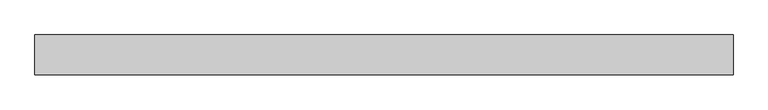
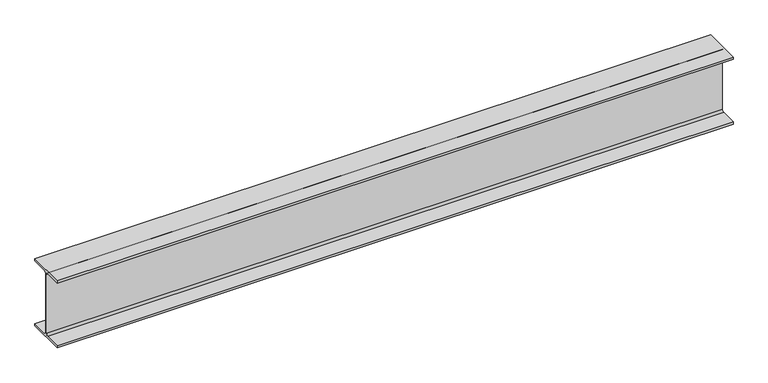
"""IFC4 building model written with IfcOpenShell, lengths in millimetres: beam geometry, Steel Beam_H-KSD3502 : H_SB_ASB_H-250x125x6x9."""

import ifcopenshell
import ifcopenshell.guid

model = None  # the IFC model being written
_history = None  # IfcOwnerHistory: only IFC2X3 demands one
_inside = {}  # id of a spatial element -> (the spatial element, [elements in it])
_under = {}  # id of a project, library or spatial element -> (it, [spatial elements below it])
_declared = {}  # id of a project -> (the project, [libraries it declares])
_typed = {}  # id of a type object -> (the type object, [elements of that type])
_made_of = {}  # id of a material, layer set ... -> (it, [elements and type objects made of it])


def new_model(schema):
    """Start an empty IFC model of exactly this schema.

    Asked for "IFC4X3", IfcOpenShell would pick the latest addendum, in which some entities
    have other attributes; the version numbers below select the first issue.
    IFC2X3 requires an IfcOwnerHistory on every rooted entity: one is made here for all.
    """
    global model, _history
    if schema == "IFC4X3":
        model = ifcopenshell.file(schema_version=(4, 3, 0, 0))
    else:
        model = ifcopenshell.file(schema=schema)
    _inside.clear()
    _under.clear()
    _declared.clear()
    _typed.clear()
    _made_of.clear()
    _history = None
    if model.schema == "IFC2X3":
        org = make("IfcOrganization", Name="unknown")
        user = make(
            "IfcPersonAndOrganization",
            ThePerson=make("IfcPerson", FamilyName="unknown"),
            TheOrganization=org,
        )
        app = make(
            "IfcApplication",
            ApplicationDeveloper=org,
            Version="unknown",
            ApplicationFullName="unknown",
            ApplicationIdentifier="unknown",
        )
        _history = make(
            "IfcOwnerHistory",
            OwningUser=user,
            OwningApplication=app,
            ChangeAction="ADDED",
            CreationDate=0,
        )
    return model


def make(cls, **values):
    """One entity of the class cls with the attributes given. An attribute that is None is left unset."""
    return model.create_entity(
        cls, **{name: value for name, value in values.items() if value is not None}
    )


def rooted(cls, **values):
    """An entity with a GlobalId (a new one), such as an element, a storey or a relation."""
    return make(cls, GlobalId=ifcopenshell.guid.new(), OwnerHistory=_history, **values)


def si_unit(unit_type, name, prefix=None):
    """IfcSIUnit, for example si_unit("LENGTHUNIT", "METRE", prefix="MILLI")."""
    return make("IfcSIUnit", UnitType=unit_type, Prefix=prefix, Name=name)


def assignment(units):
    """IfcUnitAssignment: the units of a project."""
    return None if units is None else make("IfcUnitAssignment", Units=units)


def point(xyz):
    """IfcCartesianPoint."""
    return None if xyz is None else make("IfcCartesianPoint", Coordinates=xyz)


def direction(xyz):
    """IfcDirection."""
    return None if xyz is None else make("IfcDirection", DirectionRatios=xyz)


def frame(location, z_axis=None, x_axis=None):
    """IfcAxis2Placement3D, a coordinate frame: its origin and axes. An axis left out is left unset."""
    return make(
        "IfcAxis2Placement3D",
        Location=point(location),
        Axis=direction(z_axis),
        RefDirection=direction(x_axis),
    )


def frame_2d(location, x_axis=None):
    """IfcAxis2Placement2D, a coordinate frame in the plane: its origin and x axis."""
    return make(
        "IfcAxis2Placement2D", Location=point(location), RefDirection=direction(x_axis)
    )


def origin():
    """The frame at (0, 0, 0) with its axes left unset."""
    return frame((0.0, 0.0, 0.0))


def place(relative_to, where):
    """IfcLocalPlacement: puts the frame where relative to a parent placement (None: the world)."""
    return make(
        "IfcLocalPlacement", PlacementRelTo=relative_to, RelativePlacement=where
    )


def context(
    kind, dimensions, precision=None, world=None, true_north=None, identifier=None
):
    """IfcGeometricRepresentationContext, for example the 3D "Model" context."""
    return make(
        "IfcGeometricRepresentationContext",
        ContextIdentifier=identifier,
        ContextType=kind,
        CoordinateSpaceDimension=dimensions,
        Precision=precision,
        WorldCoordinateSystem=world,
        TrueNorth=true_north,
    )


def project(units=None, contexts=None):
    """IfcProject with its units and contexts."""
    return rooted(
        "IfcProject",
        Name="project",
        RepresentationContexts=contexts,
        UnitsInContext=assignment(units),
    )


def spatial(cls, under=None, at=None, **own):
    """A site, building, storey or space (cls), placed at a placement, below another one or the project."""
    s = rooted(cls, ObjectPlacement=at, **own)
    if under is not None:
        _under.setdefault(under.id(), (under, []))[1].append(s)
    return s


def polyline(points):
    """IfcPolyline through the points."""
    return make("IfcPolyline", Points=[point(p) for p in points])


def circle_curve(where, radius):
    """IfcCircle in the frame where."""
    return make("IfcCircle", Position=where, Radius=radius)


def trimmed(basis, trim1, trim2, sense, master):
    """IfcTrimmedCurve: the piece of a basis curve between two trims."""
    return make(
        "IfcTrimmedCurve",
        BasisCurve=basis,
        Trim1=trim1,
        Trim2=trim2,
        SenseAgreement=sense,
        MasterRepresentation=master,
    )


def segment(curve, same_sense, transition):
    """IfcCompositeCurveSegment."""
    return make(
        "IfcCompositeCurveSegment",
        Transition=transition,
        SameSense=same_sense,
        ParentCurve=curve,
    )


def composite_curve(segments, self_intersect=None):
    """IfcCompositeCurve: segments joined end to end."""
    return make("IfcCompositeCurve", Segments=segments, SelfIntersect=self_intersect)


def outline(outer, holes=None, kind="AREA"):
    """IfcArbitraryClosedProfileDef: a profile drawn as a closed curve; with holes, ...WithVoids."""
    if holes is None:
        return make("IfcArbitraryClosedProfileDef", ProfileType=kind, OuterCurve=outer)
    return make(
        "IfcArbitraryProfileDefWithVoids",
        ProfileType=kind,
        OuterCurve=outer,
        InnerCurves=holes,
    )


def extrude(swept, where, along, depth):
    """IfcExtrudedAreaSolid: the profile swept, set in the frame where, extruded along a direction by depth."""
    return make(
        "IfcExtrudedAreaSolid",
        SweptArea=swept,
        Position=where,
        ExtrudedDirection=direction(along),
        Depth=depth,
    )


def shape(context_of_items, identifier, shape_type, items):
    """IfcShapeRepresentation: the items that make up one representation, for example the "Body"."""
    return make(
        "IfcShapeRepresentation",
        ContextOfItems=context_of_items,
        RepresentationIdentifier=identifier,
        RepresentationType=shape_type,
        Items=items,
    )


def source(mapping_origin, context_of_items, identifier, shape_type, items):
    """IfcRepresentationMap: a shape defined once, which mapped items show again and again."""
    return make(
        "IfcRepresentationMap",
        MappingOrigin=mapping_origin,
        MappedRepresentation=shape(context_of_items, identifier, shape_type, items),
    )


def transform(
    local_origin,
    x_axis=None,
    y_axis=None,
    z_axis=None,
    scale=None,
    scale2=None,
    scale3=None,
    uniform=True,
):
    """IfcCartesianTransformationOperator3D, or its non-uniform kind. x_axis, y_axis, z_axis: its Axis1, 2, 3."""
    if uniform:
        return make(
            "IfcCartesianTransformationOperator3D",
            Axis1=direction(x_axis),
            Axis2=direction(y_axis),
            LocalOrigin=point(local_origin),
            Scale=scale,
            Axis3=direction(z_axis),
        )
    return make(
        "IfcCartesianTransformationOperator3DnonUniform",
        Axis1=direction(x_axis),
        Axis2=direction(y_axis),
        LocalOrigin=point(local_origin),
        Scale=scale,
        Axis3=direction(z_axis),
        Scale2=scale2,
        Scale3=scale3,
    )


def mapped(mapping_source, mapping_target):
    """IfcMappedItem: shows the shape of a source again, moved by a transform."""
    return make(
        "IfcMappedItem", MappingSource=mapping_source, MappingTarget=mapping_target
    )


def made_of(thing, what):
    """Note that an element or type object is made of a material, layer set ...; save() writes the relation."""
    if what is not None:
        _made_of.setdefault(what.id(), (what, []))[1].append(thing)
    return thing


def element(
    cls,
    number,
    at=None,
    inside=None,
    cuts=None,
    type_object=None,
    material=None,
    context=None,
    identifier="Body",
    shape_type=None,
    held_by="IfcProductDefinitionShape",
    body=None,
    shapes=None,
    **own,
):
    """One element of the class cls, such as IfcWall. Its Tag is "e" and its number.

    at: its placement. inside: the storey or other place that contains it. cuts: it is an
    opening in that element (IfcRelVoidsElement). A single representation is given by context,
    identifier, shape_type and body (its items); several are given by shapes. held_by: the class
    of the entity that holds the representations. save() writes the other relations.
    """
    e = rooted(cls, Tag="e%d" % number, ObjectPlacement=at, **own)
    if body is not None:
        shapes = [shape(context, identifier, shape_type, body)]
    if shapes is not None:
        e.Representation = make(held_by, Representations=shapes)
    if inside is not None:
        _inside.setdefault(inside.id(), (inside, []))[1].append(e)
    if cuts is not None:
        rooted(
            "IfcRelVoidsElement", RelatingBuildingElement=cuts, RelatedOpeningElement=e
        )
    if type_object is not None:
        _typed.setdefault(type_object.id(), (type_object, []))[1].append(e)
    return made_of(e, material)


def aggregate(whole, parts):
    """IfcRelAggregates: a whole, such as a stair, and the parts it consists of."""
    return rooted("IfcRelAggregates", RelatingObject=whole, RelatedObjects=parts)


def save(model, path):
    """Write the relations noted so far, then the file.

    IfcRelAggregates (storeys below a building ...), IfcRelContainedInSpatialStructure (elements
    in a storey), IfcRelDefinesByType, IfcRelAssociatesMaterial and IfcRelDeclares: one each for
    every whole, place, type object, material and project.
    """
    for whole, parts in _under.values():
        aggregate(whole, parts)
    for where, things in _inside.values():
        rooted(
            "IfcRelContainedInSpatialStructure",
            RelatedElements=things,
            RelatingStructure=where,
        )
    for kind, things in _typed.values():
        rooted("IfcRelDefinesByType", RelatedObjects=things, RelatingType=kind)
    for what, things in _made_of.values():
        rooted("IfcRelAssociatesMaterial", RelatedObjects=things, RelatingMaterial=what)
    for by, libraries in _declared.values():
        rooted("IfcRelDeclares", RelatingContext=by, RelatedDefinitions=libraries)
    model.write(path)


def beam_680f737e(model_context):
    return source(origin(), model_context, "Body", "SweptSolid", [
        extrude(outline(composite_curve([segment(polyline([(82.5, -141.5), (82.5, -151.7), (-82.5, -151.7), (-82.5, -141.5), (-11.9, -141.5)]), True, "CONTINUOUS"), segment(trimmed(circle_curve(frame_2d((-11.9, -132.6)), 8.9), [point((-11.9, -141.5))], [point((-3.0, -132.6))], True, "CARTESIAN"), True, "CONTINUOUS"), segment(polyline([(-3.0, -132.6), (-3.0, 132.6)]), True, "CONTINUOUS"), segment(trimmed(circle_curve(frame_2d((-11.9, 132.6)), 8.9), [point((-3.0, 132.6))], [point((-11.9, 141.5))], True, "CARTESIAN"), True, "CONTINUOUS"), segment(polyline([(-11.9, 141.5), (-82.5, 141.5), (-82.5, 151.7), (82.5, 151.7), (82.5, 141.5), (11.9, 141.5)]), True, "CONTINUOUS"), segment(trimmed(circle_curve(frame_2d((11.9, 132.6)), 8.9), [point((11.9, 141.5))], [point((3.0, 132.6))], True, "CARTESIAN"), True, "CONTINUOUS"), segment(polyline([(3.0, 132.6), (3.0, -132.6)]), True, "CONTINUOUS"), segment(trimmed(circle_curve(frame_2d((11.9, -132.6)), 8.9), [point((3.0, -132.6))], [point((11.9, -141.5))], True, "CARTESIAN"), True, "CONTINUOUS"), segment(polyline([(11.9, -141.5), (82.5, -141.5)]), True, "CONTINUOUS")], self_intersect=False)), frame((-1404.8, 0.0, 0.0), z_axis=(1.0, 0.0, 0.0), x_axis=(0.0, 1.0, 0.0)), (0.0, 0.0, 1.0), 2892.0999994),
    ])


if __name__ == "__main__":
    model = new_model("IFC4")
    model_context = context("Model", 3, world=origin())
    ifc_project = project(units=[si_unit("LENGTHUNIT", "METRE", prefix="MILLI")], contexts=[model_context])
    site = spatial("IfcSite", under=ifc_project)
    building = spatial("IfcBuilding", under=site)
    placement = place(None, origin())
    beam_shape = beam_680f737e(model_context)
    element("IfcBeam", 1, ObjectType="Steel Beam_H-KSD3502 : H_SB_ASB_H-250x125x6x9", at=placement, inside=building, context=model_context, shape_type="MappedRepresentation", body=[
        mapped(beam_shape, transform((0.0, 0.0, 0.0), x_axis=(1.0, 0.0, 0.0), y_axis=(0.0, 1.0, 0.0), z_axis=(0.0, 0.0, 1.0))),
    ])
    save(model, "model.ifc")

# Revit data of these elements
# Type "Steel Beam_H-KSD3502 : H_SB_ASB_H-250x125x6x9"
#   Width = 12.5 cm
#   Web Thickness = 0.6 cm
#   Web Fillet = 1.2 cm
#   Warping Constant = 42539.8 cm⁶
#   Torsional Moment of Inertia = 7.8102 cm⁴
#   Torsional Modulus = 1.0 cm³
#   Section Area = 37.66 cm²
#   Plastic Modulus weak axis = 73.1 cm³
#   Plastic Modulus strong axis = 366.0 cm³
#   Perimeter = 0.97 m²/m
#   Nominal Weight = 29.60 kgf/m
#   Moment of Inertia weak axis = 294.00 cm⁴
#   Moment of Inertia strong axis = 4050.00 cm⁴
#   Height = 25.0 cm
#   Flange Thickness = 0.9 cm
#   Elastic Modulus weak axis = 47.0 cm³
#   Elastic Modulus strong axis = 324.0 cm³
#   Centroid Vertical = 12.5 cm
#   Centroid Horizontal = 6.25 cm
#   Length [instance default] = 1.5240 m
#   Structural Material [instance default] = Steel, 45-345
#   Assembly Code = ""
# Element 1 (IfcBeam, "Steel Beam_H-KSD3502 : H_SB_ASB_H-250x125x6x9")
#   Structural Material = none
# Materials
#   "Steel, 45-345": class "Metal", colour RGB 189 187 185, transparency 0, Description = "Steel 345 MPa", Cost = 0
